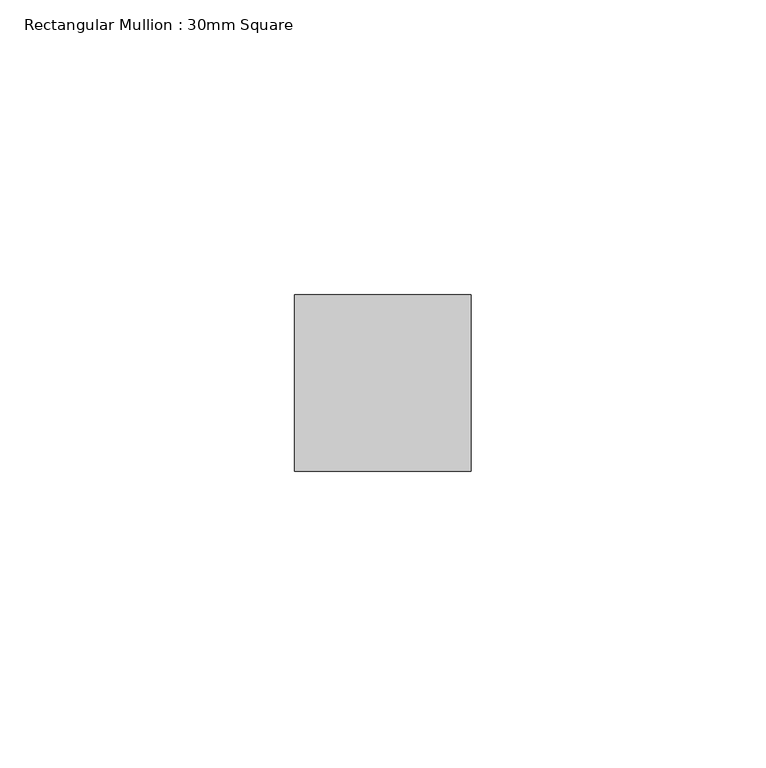
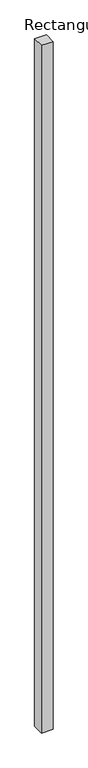
"""IFC4 building model written with IfcOpenShell, lengths in millimetres: member geometry, Rectangular Mullion : 30mm Square."""

from ifc_helpers import new_model, si_unit, frame, origin, place, context, project, spatial, polyline, outline, extrude, source, transform, mapped, element, save


def rectangular_mullion_30mm_square_c8a39bf0(model_context):
    return source(origin(), model_context, "Body", "SweptSolid", [
        extrude(outline(polyline([(15.0, 15.0), (15.0, -15.0), (-15.0, -15.0), (-15.0, 15.0), (15.0, 15.0)])), frame((0.0, 0.0, -1876.7376356), z_axis=(0.0, 0.0, 1.0), x_axis=(1.0, 0.0, 0.0)), (0.0, 0.0, 1.0), 1876.7376356),
    ])


if __name__ == "__main__":
    model = new_model("IFC4")
    model_context = context("Model", 3, world=origin())
    ifc_project = project(units=[si_unit("LENGTHUNIT", "METRE", prefix="MILLI")], contexts=[model_context])
    site = spatial("IfcSite", under=ifc_project)
    building = spatial("IfcBuilding", under=site)
    placement = place(None, origin())
    rectangular_mullion_30mm_square_shape = rectangular_mullion_30mm_square_c8a39bf0(model_context)
    element("IfcMember", 1, ObjectType="Rectangular Mullion : 30mm Square", at=placement, inside=building, context=model_context, shape_type="MappedRepresentation", body=[
        mapped(rectangular_mullion_30mm_square_shape, transform((0.0, 0.0, 0.0), x_axis=(1.0, 0.0, 0.0), y_axis=(0.0, 1.0, 0.0), z_axis=(0.0, 0.0, 1.0))),
    ])
    save(model, "model.ifc")

# Revit data of these elements
# Type "Rectangular Mullion : 30mm Square"
#   built-in parameter 1007304 = 0.0984252 (stored number, unit not read)
#   built-in parameter 1007301 = 0.0492126 (stored number, unit not read)
#   built-in parameter 1007300 = 0.0492126 (stored number, unit not read)
# Element 1 (IfcMember, "Rectangular Mullion : 30mm Square")
#   Materials on its faces: "Aluminum"
# Materials
#   "Aluminum": class "Metal", colour RGB 244 244 244, transparency 0, Description = "Aluminum 6061", Cost = 0
